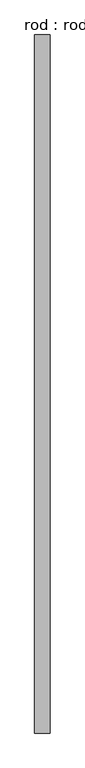
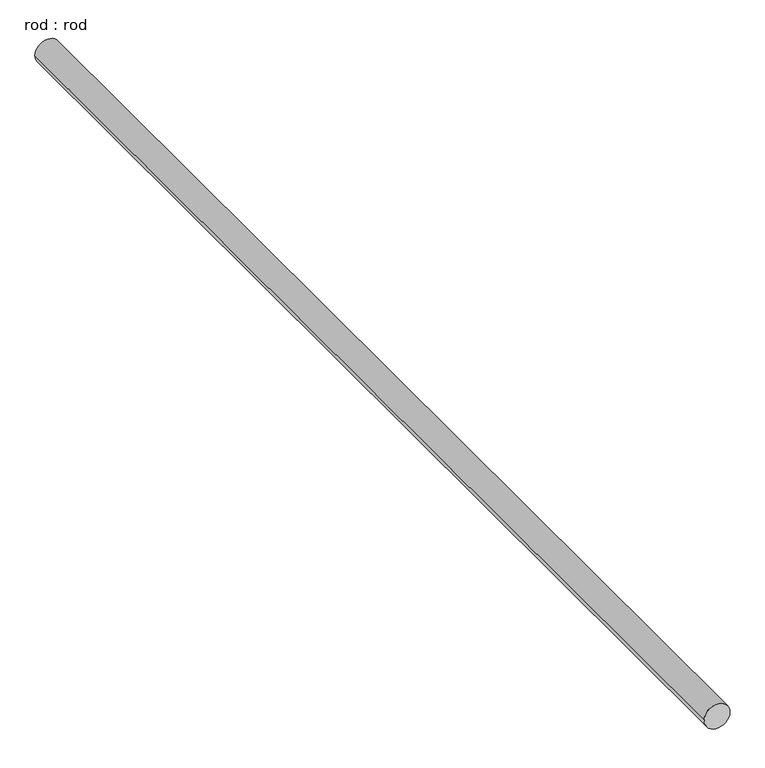
"""IFC4 building model written with IfcOpenShell, lengths in millimetres: proxy geometry, rod : rod."""

from ifc_helpers import new_model, si_unit, point, frame, frame_2d, origin, place, context, project, spatial, circle_curve, trimmed, segment, composite_curve, outline, extrude, source, transform, mapped, element, save


def rod_rod_c6649810(model_context):
    return source(origin(), model_context, "Body", "SweptSolid", [
        extrude(outline(composite_curve([segment(trimmed(circle_curve(frame_2d((0.0108462, 0.0)), 200.0), [point((0.0108462, 200.0))], [point((0.0108462, -200.0))], False, "CARTESIAN"), True, "CONTINUOUS"), segment(trimmed(circle_curve(frame_2d((0.0108462, 0.0)), 200.0), [point((0.0108462, -200.0))], [point((0.0108462, 200.0))], False, "CARTESIAN"), True, "CONTINUOUS")], self_intersect=False)), frame((0.0, -4934.0570989, 0.0), z_axis=(0.0, 1.0, 0.0), x_axis=(0.0, 0.0, 1.0)), (0.0, 0.0, 1.0), 18053.5714286),
    ])


if __name__ == "__main__":
    model = new_model("IFC4")
    model_context = context("Model", 3, world=origin())
    ifc_project = project(units=[si_unit("LENGTHUNIT", "METRE", prefix="MILLI")], contexts=[model_context])
    site = spatial("IfcSite", under=ifc_project)
    building = spatial("IfcBuilding", under=site)
    placement = place(None, origin())
    rod_rod_shape = rod_rod_c6649810(model_context)
    element("IfcBuildingElementProxy", 1, Name="rod : rod", ObjectType="rod : rod", at=placement, inside=building, context=model_context, shape_type="MappedRepresentation", body=[
        mapped(rod_rod_shape, transform((0.0, 0.0, 0.0), x_axis=(1.0, 0.0, 0.0), y_axis=(0.0, 1.0, 0.0), z_axis=(0.0, 0.0, 1.0))),
    ])
    save(model, "model.ifc")

# Revit data of these elements
# Type "rod : rod"
#   Default Elevation = 0
